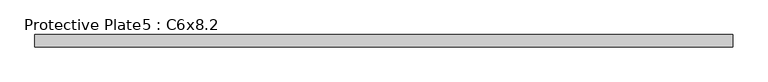
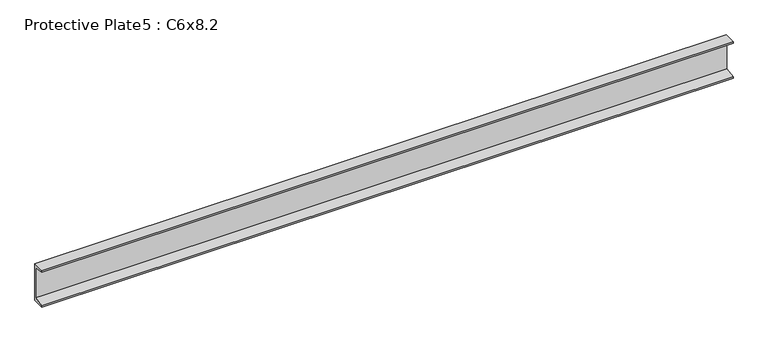
"""IFC4 building model written with IfcOpenShell, lengths in millimetres: proxy geometry, Protective Plate5 : C6x8.2."""

from ifc_helpers import new_model, si_unit, frame, origin, place, context, project, spatial, polyline, outline, extrude, source, transform, mapped, element, save


def protective_plate5_c6x8_2_0d7b6ffb(model_context):
    return source(origin(), model_context, "Body", "SweptSolid", [
        extrude(outline(polyline([(-536340.3753841, 914.4), (-536291.6073841, 914.4), (-536291.6073841, 762.0), (-536340.3753841, 762.0), (-536340.3753841, 767.08), (-536296.6675403, 774.7868721), (-536296.6675403, 901.6131279), (-536340.3753841, 909.32), (-536340.3753841, 914.4)])), frame((587467.4934739, 0.0, 0.0), z_axis=(1.0, 0.0, 0.0), x_axis=(0.0, 1.0, 0.0)), (0.0, 0.0, 1.0), 2749.55),
    ])


if __name__ == "__main__":
    model = new_model("IFC4")
    model_context = context("Model", 3, world=origin())
    ifc_project = project(units=[si_unit("LENGTHUNIT", "METRE", prefix="MILLI")], contexts=[model_context])
    site = spatial("IfcSite", under=ifc_project)
    building = spatial("IfcBuilding", under=site)
    placement = place(None, origin())
    protective_plate5_c6x8_2_shape = protective_plate5_c6x8_2_0d7b6ffb(model_context)
    element("IfcBuildingElementProxy", 1, Name="Protective Plate5 : C6x8.2", ObjectType="Protective Plate5 : C6x8.2", at=placement, inside=building, context=model_context, shape_type="MappedRepresentation", body=[
        mapped(protective_plate5_c6x8_2_shape, transform((0.0, 0.0, 0.0), x_axis=(1.0, 0.0, 0.0), y_axis=(0.0, 1.0, 0.0), z_axis=(0.0, 0.0, 1.0))),
    ])
    save(model, "model.ifc")

# Revit data of these elements
# Element 1 (IfcBuildingElementProxy, "Protective Plate5 : C6x8.2")
#   Materials on its faces: "C6x8.2 GALV CHANNEL"
# Materials
#   "C6x8.2 GALV CHANNEL": class "Generic", colour RGB 211 211 207, transparency 0, Cost = 0
